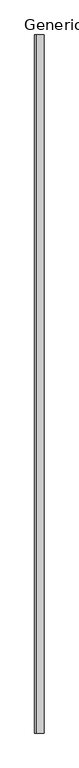
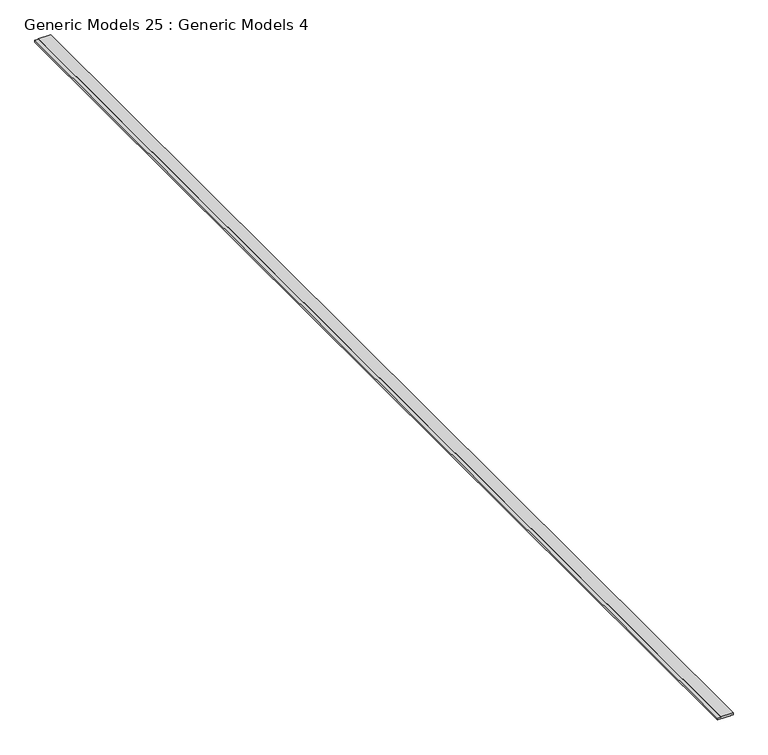
"""IFC4 building model written with IfcOpenShell, lengths in millimetres: proxy geometry, Generic Models 25 : Generic Models 4."""

from ifc_helpers import new_model, si_unit, origin, place, context, project, spatial, faceted_brep, source, transform, mapped, element, save


def generic_models_25_generic_models_4_09355143(model_context):
    return source(origin(), model_context, "Body", "Brep", [
        faceted_brep([(8583.7563705, -667.3230338, 126305.691), (8583.7563705, -667.3230338, 126317.121), (8583.7563705, -667.3230338, 126326.646), (8454.3751205, -667.3230338, 126326.646), (8454.3751205, -667.3230338, 126325.376), (8417.5451205, -667.3230338, 126325.376), (8417.5451205, -667.3230338, 126305.691), (8419.7549205, -667.3230338, 126305.691), (8419.7549205, -667.3230338, 126307.4234564), (8421.0249205, -667.3230338, 126307.4234564), (8421.0249205, -667.3230338, 126304.421), (8561.3131865, -667.3230338, 126304.421), (8561.3131865, -667.3230338, 126305.691), (8583.7563705, 11778.6769662, 126326.646), (8583.7563705, 11778.6769662, 126317.121), (8583.7563705, 11778.6769662, 126305.691), (8561.3131865, 11778.6769662, 126305.691), (8561.3131865, 11778.6769662, 126304.421), (8421.0249205, 11778.6769662, 126304.421), (8421.0249205, 11778.6769662, 126307.4234564), (8419.7549205, 11778.6769662, 126307.4234564), (8419.7549205, 11778.6769662, 126305.691), (8417.5451205, 11778.6769662, 126305.691), (8417.5451205, 11778.6769662, 126325.376), (8454.3751205, 11778.6769662, 126325.376), (8454.3751205, 11778.6769662, 126326.646)], [[[0, 1, 2, 3, 4, 5, 6, 7, 8, 9, 10, 11, 12]], [[13, 14, 15, 16, 17, 18, 19, 20, 21, 22, 23, 24, 25]], [[2, 13, 25, 3]], [[17, 11, 10, 18]], [[13, 2, 1, 0, 15, 14]], [[6, 5, 23, 22]], [[24, 4, 3, 25]], [[4, 24, 23, 5]], [[21, 7, 6, 22]], [[8, 20, 19, 9]], [[9, 19, 18, 10]], [[20, 8, 7, 21]], [[16, 12, 11, 17]], [[12, 16, 15, 0]]]),
    ])


if __name__ == "__main__":
    model = new_model("IFC4")
    model_context = context("Model", 3, world=origin())
    ifc_project = project(units=[si_unit("LENGTHUNIT", "METRE", prefix="MILLI")], contexts=[model_context])
    site = spatial("IfcSite", under=ifc_project)
    building = spatial("IfcBuilding", under=site)
    placement = place(None, origin())
    generic_models_25_generic_models_4_shape = generic_models_25_generic_models_4_09355143(model_context)
    element("IfcBuildingElementProxy", 1, Name="Generic Models 25 : Generic Models 4", ObjectType="Generic Models 25 : Generic Models 4", at=placement, inside=building, context=model_context, shape_type="MappedRepresentation", body=[
        mapped(generic_models_25_generic_models_4_shape, transform((0.0, 0.0, 0.0), x_axis=(1.0, 0.0, 0.0), y_axis=(0.0, 1.0, 0.0), z_axis=(0.0, 0.0, 1.0))),
    ])
    save(model, "model.ifc")

# Revit data of these elements
# Element 1 (IfcBuildingElementProxy, "Generic Models 25 : Generic Models 4")
#   Materials on its faces: "_7/8\" SMOOTH TROWEL EXTERIOR STUCCO (COLOR PER OWNER)"
# Materials
#   "_7/8\" SMOOTH TROWEL EXTERIOR STUCCO (COLOR PER OWNER)": class "Generic", colour RGB 233 233 233, transparency 0, Cost = 0
